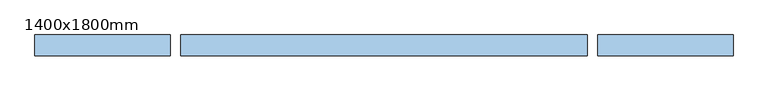
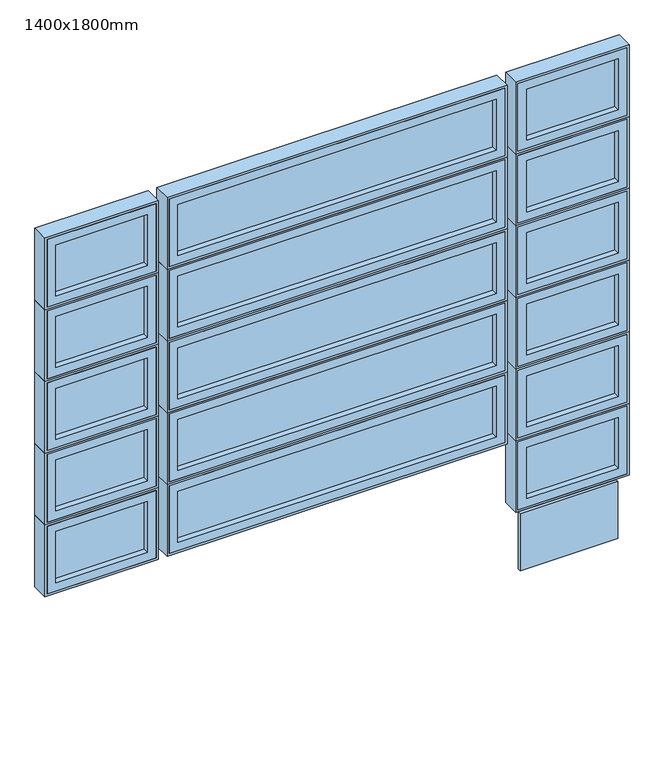
"""IFC4 building model written with IfcOpenShell, lengths in millimetres: window geometry, Janela Basculante 01 : 1400x1800mm."""

from ifc_helpers import new_model, si_unit, frame, origin, place, context, project, spatial, polyline, outline, extrude, faceted_brep, source, transform, mapped, element, save


def window_1400x1800mm_563ee437(model_context):
    return source(origin(), model_context, "Body", "SolidModel", [
        extrude(outline(polyline([(652.0, -29.6), (652.0, -36.6), (428.0, -36.6), (428.0, -29.6), (652.0, -29.6)])), frame((0.0, 0.0, 2164.0), z_axis=(0.0, 0.0, 1.0), x_axis=(1.0, 0.0, 0.0)), (0.0, 0.0, 1.0), 138.0),
        faceted_brep([(435.0, -50.6, 2295.0), (435.0, -50.6, 2171.0), (435.0, -36.6, 2171.0), (435.0, -36.6, 2295.0), (428.0, -36.6, 2302.0), (428.0, -36.6, 2164.0), (428.0, -29.6, 2164.0), (428.0, -29.6, 2302.0), (435.0, -29.6, 2295.0), (435.0, -29.6, 2171.0), (435.0, -15.6, 2171.0), (435.0, -15.6, 2295.0), (415.0, -15.6, 2315.0), (415.0, -15.6, 2151.0), (415.0, -50.6, 2151.0), (415.0, -50.6, 2315.0), (645.0, -50.6, 2171.0), (645.0, -36.6, 2171.0), (652.0, -36.6, 2164.0), (652.0, -29.6, 2164.0), (645.0, -29.6, 2171.0), (645.0, -15.6, 2171.0), (665.0, -15.6, 2151.0), (665.0, -50.6, 2151.0), (645.0, -50.6, 2295.0), (645.0, -36.6, 2295.0), (652.0, -36.6, 2302.0), (652.0, -29.6, 2302.0), (645.0, -29.6, 2295.0), (645.0, -15.6, 2295.0), (665.0, -15.6, 2315.0), (665.0, -50.6, 2315.0)], [[[0, 1, 2, 3]], [[4, 5, 6, 7]], [[8, 9, 10, 11]], [[12, 13, 14, 15]], [[1, 16, 17, 2]], [[5, 18, 19, 6]], [[9, 20, 21, 10]], [[13, 22, 23, 14]], [[16, 24, 25, 17]], [[18, 26, 27, 19]], [[20, 28, 29, 21]], [[22, 30, 31, 23]], [[15, 14, 23, 31], [1, 0, 24, 16]], [[24, 0, 3, 25]], [[5, 4, 26, 18], [3, 2, 17, 25]], [[26, 4, 7, 27]], [[7, 6, 19, 27], [9, 8, 28, 20]], [[28, 8, 11, 29]], [[13, 12, 30, 22], [11, 10, 21, 29]], [[30, 12, 15, 31]]]),
        faceted_brep([(415.0, -50.6, 2315.0), (415.0, -50.6, 2151.0), (415.0, -15.6, 2151.0), (415.0, -15.6, 2315.0), (420.0, -15.6, 2310.0), (420.0, -15.6, 2156.0), (420.0, -10.6, 2156.0), (420.0, -10.6, 2310.0), (410.0, -10.6, 2320.0), (410.0, -10.6, 2146.0), (410.0, -50.6, 2146.0), (410.0, -50.6, 2320.0), (665.0, -50.6, 2151.0), (665.0, -15.6, 2151.0), (660.0, -15.6, 2156.0), (660.0, -10.6, 2156.0), (670.0, -10.6, 2146.0), (670.0, -50.6, 2146.0), (665.0, -50.6, 2315.0), (665.0, -15.6, 2315.0), (660.0, -15.6, 2310.0), (660.0, -10.6, 2310.0), (670.0, -10.6, 2320.0), (670.0, -50.6, 2320.0)], [[[0, 1, 2, 3]], [[4, 5, 6, 7]], [[8, 9, 10, 11]], [[1, 12, 13, 2]], [[5, 14, 15, 6]], [[9, 16, 17, 10]], [[12, 18, 19, 13]], [[14, 20, 21, 15]], [[16, 22, 23, 17]], [[11, 10, 17, 23], [1, 0, 18, 12]], [[18, 0, 3, 19]], [[3, 2, 13, 19], [5, 4, 20, 14]], [[20, 4, 7, 21]], [[9, 8, 22, 16], [7, 6, 15, 21]], [[22, 8, 11, 23]]]),
        extrude(outline(polyline([(652.0, -29.6), (652.0, -36.6), (428.0, -36.6), (428.0, -29.6), (652.0, -29.6)])), frame((0.0, 0.0, 1990.0), z_axis=(0.0, 0.0, 1.0), x_axis=(1.0, 0.0, 0.0)), (0.0, 0.0, 1.0), 138.0),
        faceted_brep([(435.0, -50.6, 2121.0), (435.0, -50.6, 1997.0), (435.0, -36.6, 1997.0), (435.0, -36.6, 2121.0), (428.0, -36.6, 2128.0), (428.0, -36.6, 1990.0), (428.0, -29.6, 1990.0), (428.0, -29.6, 2128.0), (435.0, -29.6, 2121.0), (435.0, -29.6, 1997.0), (435.0, -15.6, 1997.0), (435.0, -15.6, 2121.0), (415.0, -15.6, 2141.0), (415.0, -15.6, 1977.0), (415.0, -50.6, 1977.0), (415.0, -50.6, 2141.0), (645.0, -50.6, 1997.0), (645.0, -36.6, 1997.0), (652.0, -36.6, 1990.0), (652.0, -29.6, 1990.0), (645.0, -29.6, 1997.0), (645.0, -15.6, 1997.0), (665.0, -15.6, 1977.0), (665.0, -50.6, 1977.0), (645.0, -50.6, 2121.0), (645.0, -36.6, 2121.0), (652.0, -36.6, 2128.0), (652.0, -29.6, 2128.0), (645.0, -29.6, 2121.0), (645.0, -15.6, 2121.0), (665.0, -15.6, 2141.0), (665.0, -50.6, 2141.0)], [[[0, 1, 2, 3]], [[4, 5, 6, 7]], [[8, 9, 10, 11]], [[12, 13, 14, 15]], [[1, 16, 17, 2]], [[5, 18, 19, 6]], [[9, 20, 21, 10]], [[13, 22, 23, 14]], [[16, 24, 25, 17]], [[18, 26, 27, 19]], [[20, 28, 29, 21]], [[22, 30, 31, 23]], [[15, 14, 23, 31], [1, 0, 24, 16]], [[24, 0, 3, 25]], [[5, 4, 26, 18], [3, 2, 17, 25]], [[26, 4, 7, 27]], [[7, 6, 19, 27], [9, 8, 28, 20]], [[28, 8, 11, 29]], [[13, 12, 30, 22], [11, 10, 21, 29]], [[30, 12, 15, 31]]]),
        faceted_brep([(415.0, -50.6, 2141.0), (415.0, -50.6, 1977.0), (415.0, -15.6, 1977.0), (415.0, -15.6, 2141.0), (420.0, -15.6, 2136.0), (420.0, -15.6, 1982.0), (420.0, -10.6, 1982.0), (420.0, -10.6, 2136.0), (410.0, -10.6, 2146.0), (410.0, -10.6, 1972.0), (410.0, -50.6, 1972.0), (410.0, -50.6, 2146.0), (665.0, -50.6, 1977.0), (665.0, -15.6, 1977.0), (660.0, -15.6, 1982.0), (660.0, -10.6, 1982.0), (670.0, -10.6, 1972.0), (670.0, -50.6, 1972.0), (665.0, -50.6, 2141.0), (665.0, -15.6, 2141.0), (660.0, -15.6, 2136.0), (660.0, -10.6, 2136.0), (670.0, -10.6, 2146.0), (670.0, -50.6, 2146.0)], [[[0, 1, 2, 3]], [[4, 5, 6, 7]], [[8, 9, 10, 11]], [[1, 12, 13, 2]], [[5, 14, 15, 6]], [[9, 16, 17, 10]], [[12, 18, 19, 13]], [[14, 20, 21, 15]], [[16, 22, 23, 17]], [[11, 10, 17, 23], [1, 0, 18, 12]], [[18, 0, 3, 19]], [[3, 2, 13, 19], [5, 4, 20, 14]], [[20, 4, 7, 21]], [[9, 8, 22, 16], [7, 6, 15, 21]], [[22, 8, 11, 23]]]),
        extrude(outline(polyline([(652.0, -29.6), (652.0, -36.6), (428.0, -36.6), (428.0, -29.6), (652.0, -29.6)])), frame((0.0, 0.0, 1816.0), z_axis=(0.0, 0.0, 1.0), x_axis=(1.0, 0.0, 0.0)), (0.0, 0.0, 1.0), 138.0),
        faceted_brep([(435.0, -50.6, 1947.0), (435.0, -50.6, 1823.0), (435.0, -36.6, 1823.0), (435.0, -36.6, 1947.0), (428.0, -36.6, 1954.0), (428.0, -36.6, 1816.0), (428.0, -29.6, 1816.0), (428.0, -29.6, 1954.0), (435.0, -29.6, 1947.0), (435.0, -29.6, 1823.0), (435.0, -15.6, 1823.0), (435.0, -15.6, 1947.0), (415.0, -15.6, 1967.0), (415.0, -15.6, 1803.0), (415.0, -50.6, 1803.0), (415.0, -50.6, 1967.0), (645.0, -50.6, 1823.0), (645.0, -36.6, 1823.0), (652.0, -36.6, 1816.0), (652.0, -29.6, 1816.0), (645.0, -29.6, 1823.0), (645.0, -15.6, 1823.0), (665.0, -15.6, 1803.0), (665.0, -50.6, 1803.0), (645.0, -50.6, 1947.0), (645.0, -36.6, 1947.0), (652.0, -36.6, 1954.0), (652.0, -29.6, 1954.0), (645.0, -29.6, 1947.0), (645.0, -15.6, 1947.0), (665.0, -15.6, 1967.0), (665.0, -50.6, 1967.0)], [[[0, 1, 2, 3]], [[4, 5, 6, 7]], [[8, 9, 10, 11]], [[12, 13, 14, 15]], [[1, 16, 17, 2]], [[5, 18, 19, 6]], [[9, 20, 21, 10]], [[13, 22, 23, 14]], [[16, 24, 25, 17]], [[18, 26, 27, 19]], [[20, 28, 29, 21]], [[22, 30, 31, 23]], [[15, 14, 23, 31], [1, 0, 24, 16]], [[24, 0, 3, 25]], [[5, 4, 26, 18], [3, 2, 17, 25]], [[26, 4, 7, 27]], [[7, 6, 19, 27], [9, 8, 28, 20]], [[28, 8, 11, 29]], [[13, 12, 30, 22], [11, 10, 21, 29]], [[30, 12, 15, 31]]]),
        faceted_brep([(415.0, -50.6, 1967.0), (415.0, -50.6, 1803.0), (415.0, -15.6, 1803.0), (415.0, -15.6, 1967.0), (420.0, -15.6, 1962.0), (420.0, -15.6, 1808.0), (420.0, -10.6, 1808.0), (420.0, -10.6, 1962.0), (410.0, -10.6, 1972.0), (410.0, -10.6, 1798.0), (410.0, -50.6, 1798.0), (410.0, -50.6, 1972.0), (665.0, -50.6, 1803.0), (665.0, -15.6, 1803.0), (660.0, -15.6, 1808.0), (660.0, -10.6, 1808.0), (670.0, -10.6, 1798.0), (670.0, -50.6, 1798.0), (665.0, -50.6, 1967.0), (665.0, -15.6, 1967.0), (660.0, -15.6, 1962.0), (660.0, -10.6, 1962.0), (670.0, -10.6, 1972.0), (670.0, -50.6, 1972.0)], [[[0, 1, 2, 3]], [[4, 5, 6, 7]], [[8, 9, 10, 11]], [[1, 12, 13, 2]], [[5, 14, 15, 6]], [[9, 16, 17, 10]], [[12, 18, 19, 13]], [[14, 20, 21, 15]], [[16, 22, 23, 17]], [[11, 10, 17, 23], [1, 0, 18, 12]], [[18, 0, 3, 19]], [[3, 2, 13, 19], [5, 4, 20, 14]], [[20, 4, 7, 21]], [[9, 8, 22, 16], [7, 6, 15, 21]], [[22, 8, 11, 23]]]),
        extrude(outline(polyline([(-372.0, -29.6), (372.0, -29.6), (372.0, -36.6), (-372.0, -36.6), (-372.0, -29.6)])), frame((0.0, 0.0, 2164.0), z_axis=(0.0, 0.0, 1.0), x_axis=(1.0, 0.0, 0.0)), (0.0, 0.0, 1.0), 138.0),
        faceted_brep([(365.0, -50.6, 2295.0), (365.0, -36.6, 2295.0), (365.0, -36.6, 2171.0), (365.0, -50.6, 2171.0), (372.0, -36.6, 2302.0), (372.0, -29.6, 2302.0), (372.0, -29.6, 2164.0), (372.0, -36.6, 2164.0), (365.0, -29.6, 2295.0), (365.0, -15.6, 2295.0), (365.0, -15.6, 2171.0), (365.0, -29.6, 2171.0), (385.0, -15.6, 2315.0), (385.0, -50.6, 2315.0), (385.0, -50.6, 2151.0), (385.0, -15.6, 2151.0), (-365.0, -36.6, 2171.0), (-365.0, -50.6, 2171.0), (-372.0, -29.6, 2164.0), (-372.0, -36.6, 2164.0), (-365.0, -15.6, 2171.0), (-365.0, -29.6, 2171.0), (-385.0, -50.6, 2151.0), (-385.0, -15.6, 2151.0), (-365.0, -36.6, 2295.0), (-365.0, -50.6, 2295.0), (-372.0, -29.6, 2302.0), (-372.0, -36.6, 2302.0), (-365.0, -15.6, 2295.0), (-365.0, -29.6, 2295.0), (-385.0, -50.6, 2315.0), (-385.0, -15.6, 2315.0)], [[[0, 1, 2, 3]], [[4, 5, 6, 7]], [[8, 9, 10, 11]], [[12, 13, 14, 15]], [[3, 2, 16, 17]], [[7, 6, 18, 19]], [[11, 10, 20, 21]], [[15, 14, 22, 23]], [[17, 16, 24, 25]], [[19, 18, 26, 27]], [[21, 20, 28, 29]], [[23, 22, 30, 31]], [[13, 30, 22, 14], [3, 17, 25, 0]], [[25, 24, 1, 0]], [[7, 19, 27, 4], [1, 24, 16, 2]], [[27, 26, 5, 4]], [[5, 26, 18, 6], [11, 21, 29, 8]], [[29, 28, 9, 8]], [[15, 23, 31, 12], [9, 28, 20, 10]], [[31, 30, 13, 12]]]),
        faceted_brep([(385.0, -50.6, 2315.0), (385.0, -15.6, 2315.0), (385.0, -15.6, 2151.0), (385.0, -50.6, 2151.0), (380.0, -15.6, 2310.0), (380.0, -10.6, 2310.0), (380.0, -10.6, 2156.0), (380.0, -15.6, 2156.0), (390.0, -10.6, 2320.0), (390.0, -50.6, 2320.0), (390.0, -50.6, 2146.0), (390.0, -10.6, 2146.0), (-385.0, -15.6, 2151.0), (-385.0, -50.6, 2151.0), (-380.0, -10.6, 2156.0), (-380.0, -15.6, 2156.0), (-390.0, -50.6, 2146.0), (-390.0, -10.6, 2146.0), (-385.0, -15.6, 2315.0), (-385.0, -50.6, 2315.0), (-380.0, -10.6, 2310.0), (-380.0, -15.6, 2310.0), (-390.0, -50.6, 2320.0), (-390.0, -10.6, 2320.0)], [[[0, 1, 2, 3]], [[4, 5, 6, 7]], [[8, 9, 10, 11]], [[3, 2, 12, 13]], [[7, 6, 14, 15]], [[11, 10, 16, 17]], [[13, 12, 18, 19]], [[15, 14, 20, 21]], [[17, 16, 22, 23]], [[9, 22, 16, 10], [3, 13, 19, 0]], [[19, 18, 1, 0]], [[1, 18, 12, 2], [7, 15, 21, 4]], [[21, 20, 5, 4]], [[11, 17, 23, 8], [5, 20, 14, 6]], [[23, 22, 9, 8]]]),
        extrude(outline(polyline([(-372.0, -29.6), (372.0, -29.6), (372.0, -36.6), (-372.0, -36.6), (-372.0, -29.6)])), frame((0.0, 0.0, 1990.0), z_axis=(0.0, 0.0, 1.0), x_axis=(1.0, 0.0, 0.0)), (0.0, 0.0, 1.0), 138.0),
        faceted_brep([(365.0, -50.6, 2121.0), (365.0, -36.6, 2121.0), (365.0, -36.6, 1997.0), (365.0, -50.6, 1997.0), (372.0, -36.6, 2128.0), (372.0, -29.6, 2128.0), (372.0, -29.6, 1990.0), (372.0, -36.6, 1990.0), (365.0, -29.6, 2121.0), (365.0, -15.6, 2121.0), (365.0, -15.6, 1997.0), (365.0, -29.6, 1997.0), (385.0, -15.6, 2141.0), (385.0, -50.6, 2141.0), (385.0, -50.6, 1977.0), (385.0, -15.6, 1977.0), (-365.0, -36.6, 1997.0), (-365.0, -50.6, 1997.0), (-372.0, -29.6, 1990.0), (-372.0, -36.6, 1990.0), (-365.0, -15.6, 1997.0), (-365.0, -29.6, 1997.0), (-385.0, -50.6, 1977.0), (-385.0, -15.6, 1977.0), (-365.0, -36.6, 2121.0), (-365.0, -50.6, 2121.0), (-372.0, -29.6, 2128.0), (-372.0, -36.6, 2128.0), (-365.0, -15.6, 2121.0), (-365.0, -29.6, 2121.0), (-385.0, -50.6, 2141.0), (-385.0, -15.6, 2141.0)], [[[0, 1, 2, 3]], [[4, 5, 6, 7]], [[8, 9, 10, 11]], [[12, 13, 14, 15]], [[3, 2, 16, 17]], [[7, 6, 18, 19]], [[11, 10, 20, 21]], [[15, 14, 22, 23]], [[17, 16, 24, 25]], [[19, 18, 26, 27]], [[21, 20, 28, 29]], [[23, 22, 30, 31]], [[13, 30, 22, 14], [3, 17, 25, 0]], [[25, 24, 1, 0]], [[7, 19, 27, 4], [1, 24, 16, 2]], [[27, 26, 5, 4]], [[5, 26, 18, 6], [11, 21, 29, 8]], [[29, 28, 9, 8]], [[15, 23, 31, 12], [9, 28, 20, 10]], [[31, 30, 13, 12]]]),
        faceted_brep([(385.0, -50.6, 2141.0), (385.0, -15.6, 2141.0), (385.0, -15.6, 1977.0), (385.0, -50.6, 1977.0), (380.0, -15.6, 2136.0), (380.0, -10.6, 2136.0), (380.0, -10.6, 1982.0), (380.0, -15.6, 1982.0), (390.0, -10.6, 2146.0), (390.0, -50.6, 2146.0), (390.0, -50.6, 1972.0), (390.0, -10.6, 1972.0), (-385.0, -15.6, 1977.0), (-385.0, -50.6, 1977.0), (-380.0, -10.6, 1982.0), (-380.0, -15.6, 1982.0), (-390.0, -50.6, 1972.0), (-390.0, -10.6, 1972.0), (-385.0, -15.6, 2141.0), (-385.0, -50.6, 2141.0), (-380.0, -10.6, 2136.0), (-380.0, -15.6, 2136.0), (-390.0, -50.6, 2146.0), (-390.0, -10.6, 2146.0)], [[[0, 1, 2, 3]], [[4, 5, 6, 7]], [[8, 9, 10, 11]], [[3, 2, 12, 13]], [[7, 6, 14, 15]], [[11, 10, 16, 17]], [[13, 12, 18, 19]], [[15, 14, 20, 21]], [[17, 16, 22, 23]], [[9, 22, 16, 10], [3, 13, 19, 0]], [[19, 18, 1, 0]], [[1, 18, 12, 2], [7, 15, 21, 4]], [[21, 20, 5, 4]], [[11, 17, 23, 8], [5, 20, 14, 6]], [[23, 22, 9, 8]]]),
        extrude(outline(polyline([(-372.0, -29.6), (372.0, -29.6), (372.0, -36.6), (-372.0, -36.6), (-372.0, -29.6)])), frame((0.0, 0.0, 1816.0), z_axis=(0.0, 0.0, 1.0), x_axis=(1.0, 0.0, 0.0)), (0.0, 0.0, 1.0), 138.0),
        faceted_brep([(365.0, -50.6, 1947.0), (365.0, -36.6, 1947.0), (365.0, -36.6, 1823.0), (365.0, -50.6, 1823.0), (372.0, -36.6, 1954.0), (372.0, -29.6, 1954.0), (372.0, -29.6, 1816.0), (372.0, -36.6, 1816.0), (365.0, -29.6, 1947.0), (365.0, -15.6, 1947.0), (365.0, -15.6, 1823.0), (365.0, -29.6, 1823.0), (385.0, -15.6, 1967.0), (385.0, -50.6, 1967.0), (385.0, -50.6, 1803.0), (385.0, -15.6, 1803.0), (-365.0, -36.6, 1823.0), (-365.0, -50.6, 1823.0), (-372.0, -29.6, 1816.0), (-372.0, -36.6, 1816.0), (-365.0, -15.6, 1823.0), (-365.0, -29.6, 1823.0), (-385.0, -50.6, 1803.0), (-385.0, -15.6, 1803.0), (-365.0, -36.6, 1947.0), (-365.0, -50.6, 1947.0), (-372.0, -29.6, 1954.0), (-372.0, -36.6, 1954.0), (-365.0, -15.6, 1947.0), (-365.0, -29.6, 1947.0), (-385.0, -50.6, 1967.0), (-385.0, -15.6, 1967.0)], [[[0, 1, 2, 3]], [[4, 5, 6, 7]], [[8, 9, 10, 11]], [[12, 13, 14, 15]], [[3, 2, 16, 17]], [[7, 6, 18, 19]], [[11, 10, 20, 21]], [[15, 14, 22, 23]], [[17, 16, 24, 25]], [[19, 18, 26, 27]], [[21, 20, 28, 29]], [[23, 22, 30, 31]], [[13, 30, 22, 14], [3, 17, 25, 0]], [[25, 24, 1, 0]], [[7, 19, 27, 4], [1, 24, 16, 2]], [[27, 26, 5, 4]], [[5, 26, 18, 6], [11, 21, 29, 8]], [[29, 28, 9, 8]], [[15, 23, 31, 12], [9, 28, 20, 10]], [[31, 30, 13, 12]]]),
        faceted_brep([(385.0, -50.6, 1967.0), (385.0, -15.6, 1967.0), (385.0, -15.6, 1803.0), (385.0, -50.6, 1803.0), (380.0, -15.6, 1962.0), (380.0, -10.6, 1962.0), (380.0, -10.6, 1808.0), (380.0, -15.6, 1808.0), (390.0, -10.6, 1972.0), (390.0, -50.6, 1972.0), (390.0, -50.6, 1798.0), (390.0, -10.6, 1798.0), (-385.0, -15.6, 1803.0), (-385.0, -50.6, 1803.0), (-380.0, -10.6, 1808.0), (-380.0, -15.6, 1808.0), (-390.0, -50.6, 1798.0), (-390.0, -10.6, 1798.0), (-385.0, -15.6, 1967.0), (-385.0, -50.6, 1967.0), (-380.0, -10.6, 1962.0), (-380.0, -15.6, 1962.0), (-390.0, -50.6, 1972.0), (-390.0, -10.6, 1972.0)], [[[0, 1, 2, 3]], [[4, 5, 6, 7]], [[8, 9, 10, 11]], [[3, 2, 12, 13]], [[7, 6, 14, 15]], [[11, 10, 16, 17]], [[13, 12, 18, 19]], [[15, 14, 20, 21]], [[17, 16, 22, 23]], [[9, 22, 16, 10], [3, 13, 19, 0]], [[19, 18, 1, 0]], [[1, 18, 12, 2], [7, 15, 21, 4]], [[21, 20, 5, 4]], [[11, 17, 23, 8], [5, 20, 14, 6]], [[23, 22, 9, 8]]]),
        extrude(outline(polyline([(-428.0, -29.6), (-428.0, -36.6), (-652.0, -36.6), (-652.0, -29.6), (-428.0, -29.6)])), frame((0.0, 0.0, 2164.0), z_axis=(0.0, 0.0, 1.0), x_axis=(1.0, 0.0, 0.0)), (0.0, 0.0, 1.0), 138.0),
        faceted_brep([(-645.0, -50.6, 2295.0), (-645.0, -50.6, 2171.0), (-645.0, -36.6, 2171.0), (-645.0, -36.6, 2295.0), (-652.0, -36.6, 2302.0), (-652.0, -36.6, 2164.0), (-652.0, -29.6, 2164.0), (-652.0, -29.6, 2302.0), (-645.0, -29.6, 2295.0), (-645.0, -29.6, 2171.0), (-645.0, -15.6, 2171.0), (-645.0, -15.6, 2295.0), (-665.0, -15.6, 2315.0), (-665.0, -15.6, 2151.0), (-665.0, -50.6, 2151.0), (-665.0, -50.6, 2315.0), (-435.0, -50.6, 2171.0), (-435.0, -36.6, 2171.0), (-428.0, -36.6, 2164.0), (-428.0, -29.6, 2164.0), (-435.0, -29.6, 2171.0), (-435.0, -15.6, 2171.0), (-415.0, -15.6, 2151.0), (-415.0, -50.6, 2151.0), (-435.0, -50.6, 2295.0), (-435.0, -36.6, 2295.0), (-428.0, -36.6, 2302.0), (-428.0, -29.6, 2302.0), (-435.0, -29.6, 2295.0), (-435.0, -15.6, 2295.0), (-415.0, -15.6, 2315.0), (-415.0, -50.6, 2315.0)], [[[0, 1, 2, 3]], [[4, 5, 6, 7]], [[8, 9, 10, 11]], [[12, 13, 14, 15]], [[1, 16, 17, 2]], [[5, 18, 19, 6]], [[9, 20, 21, 10]], [[13, 22, 23, 14]], [[16, 24, 25, 17]], [[18, 26, 27, 19]], [[20, 28, 29, 21]], [[22, 30, 31, 23]], [[15, 14, 23, 31], [1, 0, 24, 16]], [[24, 0, 3, 25]], [[5, 4, 26, 18], [3, 2, 17, 25]], [[26, 4, 7, 27]], [[7, 6, 19, 27], [9, 8, 28, 20]], [[28, 8, 11, 29]], [[13, 12, 30, 22], [11, 10, 21, 29]], [[30, 12, 15, 31]]]),
        faceted_brep([(-665.0, -50.6, 2315.0), (-665.0, -50.6, 2151.0), (-665.0, -15.6, 2151.0), (-665.0, -15.6, 2315.0), (-660.0, -15.6, 2310.0), (-660.0, -15.6, 2156.0), (-660.0, -10.6, 2156.0), (-660.0, -10.6, 2310.0), (-670.0, -10.6, 2320.0), (-670.0, -10.6, 2146.0), (-670.0, -50.6, 2146.0), (-670.0, -50.6, 2320.0), (-415.0, -50.6, 2151.0), (-415.0, -15.6, 2151.0), (-420.0, -15.6, 2156.0), (-420.0, -10.6, 2156.0), (-410.0, -10.6, 2146.0), (-410.0, -50.6, 2146.0), (-415.0, -50.6, 2315.0), (-415.0, -15.6, 2315.0), (-420.0, -15.6, 2310.0), (-420.0, -10.6, 2310.0), (-410.0, -10.6, 2320.0), (-410.0, -50.6, 2320.0)], [[[0, 1, 2, 3]], [[4, 5, 6, 7]], [[8, 9, 10, 11]], [[1, 12, 13, 2]], [[5, 14, 15, 6]], [[9, 16, 17, 10]], [[12, 18, 19, 13]], [[14, 20, 21, 15]], [[16, 22, 23, 17]], [[11, 10, 17, 23], [1, 0, 18, 12]], [[18, 0, 3, 19]], [[3, 2, 13, 19], [5, 4, 20, 14]], [[20, 4, 7, 21]], [[9, 8, 22, 16], [7, 6, 15, 21]], [[22, 8, 11, 23]]]),
        extrude(outline(polyline([(-428.0, -29.6), (-428.0, -36.6), (-652.0, -36.6), (-652.0, -29.6), (-428.0, -29.6)])), frame((0.0, 0.0, 1990.0), z_axis=(0.0, 0.0, 1.0), x_axis=(1.0, 0.0, 0.0)), (0.0, 0.0, 1.0), 138.0),
        faceted_brep([(-645.0, -50.6, 2121.0), (-645.0, -50.6, 1997.0), (-645.0, -36.6, 1997.0), (-645.0, -36.6, 2121.0), (-652.0, -36.6, 2128.0), (-652.0, -36.6, 1990.0), (-652.0, -29.6, 1990.0), (-652.0, -29.6, 2128.0), (-645.0, -29.6, 2121.0), (-645.0, -29.6, 1997.0), (-645.0, -15.6, 1997.0), (-645.0, -15.6, 2121.0), (-665.0, -15.6, 2141.0), (-665.0, -15.6, 1977.0), (-665.0, -50.6, 1977.0), (-665.0, -50.6, 2141.0), (-435.0, -50.6, 1997.0), (-435.0, -36.6, 1997.0), (-428.0, -36.6, 1990.0), (-428.0, -29.6, 1990.0), (-435.0, -29.6, 1997.0), (-435.0, -15.6, 1997.0), (-415.0, -15.6, 1977.0), (-415.0, -50.6, 1977.0), (-435.0, -50.6, 2121.0), (-435.0, -36.6, 2121.0), (-428.0, -36.6, 2128.0), (-428.0, -29.6, 2128.0), (-435.0, -29.6, 2121.0), (-435.0, -15.6, 2121.0), (-415.0, -15.6, 2141.0), (-415.0, -50.6, 2141.0)], [[[0, 1, 2, 3]], [[4, 5, 6, 7]], [[8, 9, 10, 11]], [[12, 13, 14, 15]], [[1, 16, 17, 2]], [[5, 18, 19, 6]], [[9, 20, 21, 10]], [[13, 22, 23, 14]], [[16, 24, 25, 17]], [[18, 26, 27, 19]], [[20, 28, 29, 21]], [[22, 30, 31, 23]], [[15, 14, 23, 31], [1, 0, 24, 16]], [[24, 0, 3, 25]], [[5, 4, 26, 18], [3, 2, 17, 25]], [[26, 4, 7, 27]], [[7, 6, 19, 27], [9, 8, 28, 20]], [[28, 8, 11, 29]], [[13, 12, 30, 22], [11, 10, 21, 29]], [[30, 12, 15, 31]]]),
        faceted_brep([(-665.0, -50.6, 2141.0), (-665.0, -50.6, 1977.0), (-665.0, -15.6, 1977.0), (-665.0, -15.6, 2141.0), (-660.0, -15.6, 2136.0), (-660.0, -15.6, 1982.0), (-660.0, -10.6, 1982.0), (-660.0, -10.6, 2136.0), (-670.0, -10.6, 2146.0), (-670.0, -10.6, 1972.0), (-670.0, -50.6, 1972.0), (-670.0, -50.6, 2146.0), (-415.0, -50.6, 1977.0), (-415.0, -15.6, 1977.0), (-420.0, -15.6, 1982.0), (-420.0, -10.6, 1982.0), (-410.0, -10.6, 1972.0), (-410.0, -50.6, 1972.0), (-415.0, -50.6, 2141.0), (-415.0, -15.6, 2141.0), (-420.0, -15.6, 2136.0), (-420.0, -10.6, 2136.0), (-410.0, -10.6, 2146.0), (-410.0, -50.6, 2146.0)], [[[0, 1, 2, 3]], [[4, 5, 6, 7]], [[8, 9, 10, 11]], [[1, 12, 13, 2]], [[5, 14, 15, 6]], [[9, 16, 17, 10]], [[12, 18, 19, 13]], [[14, 20, 21, 15]], [[16, 22, 23, 17]], [[11, 10, 17, 23], [1, 0, 18, 12]], [[18, 0, 3, 19]], [[3, 2, 13, 19], [5, 4, 20, 14]], [[20, 4, 7, 21]], [[9, 8, 22, 16], [7, 6, 15, 21]], [[22, 8, 11, 23]]]),
        extrude(outline(polyline([(-428.0, -29.6), (-428.0, -36.6), (-652.0, -36.6), (-652.0, -29.6), (-428.0, -29.6)])), frame((0.0, 0.0, 1816.0), z_axis=(0.0, 0.0, 1.0), x_axis=(1.0, 0.0, 0.0)), (0.0, 0.0, 1.0), 138.0),
        faceted_brep([(-645.0, -50.6, 1947.0), (-645.0, -50.6, 1823.0), (-645.0, -36.6, 1823.0), (-645.0, -36.6, 1947.0), (-652.0, -36.6, 1954.0), (-652.0, -36.6, 1816.0), (-652.0, -29.6, 1816.0), (-652.0, -29.6, 1954.0), (-645.0, -29.6, 1947.0), (-645.0, -29.6, 1823.0), (-645.0, -15.6, 1823.0), (-645.0, -15.6, 1947.0), (-665.0, -15.6, 1967.0), (-665.0, -15.6, 1803.0), (-665.0, -50.6, 1803.0), (-665.0, -50.6, 1967.0), (-435.0, -50.6, 1823.0), (-435.0, -36.6, 1823.0), (-428.0, -36.6, 1816.0), (-428.0, -29.6, 1816.0), (-435.0, -29.6, 1823.0), (-435.0, -15.6, 1823.0), (-415.0, -15.6, 1803.0), (-415.0, -50.6, 1803.0), (-435.0, -50.6, 1947.0), (-435.0, -36.6, 1947.0), (-428.0, -36.6, 1954.0), (-428.0, -29.6, 1954.0), (-435.0, -29.6, 1947.0), (-435.0, -15.6, 1947.0), (-415.0, -15.6, 1967.0), (-415.0, -50.6, 1967.0)], [[[0, 1, 2, 3]], [[4, 5, 6, 7]], [[8, 9, 10, 11]], [[12, 13, 14, 15]], [[1, 16, 17, 2]], [[5, 18, 19, 6]], [[9, 20, 21, 10]], [[13, 22, 23, 14]], [[16, 24, 25, 17]], [[18, 26, 27, 19]], [[20, 28, 29, 21]], [[22, 30, 31, 23]], [[15, 14, 23, 31], [1, 0, 24, 16]], [[24, 0, 3, 25]], [[5, 4, 26, 18], [3, 2, 17, 25]], [[26, 4, 7, 27]], [[7, 6, 19, 27], [9, 8, 28, 20]], [[28, 8, 11, 29]], [[13, 12, 30, 22], [11, 10, 21, 29]], [[30, 12, 15, 31]]]),
        faceted_brep([(-665.0, -50.6, 1967.0), (-665.0, -50.6, 1803.0), (-665.0, -15.6, 1803.0), (-665.0, -15.6, 1967.0), (-660.0, -15.6, 1962.0), (-660.0, -15.6, 1808.0), (-660.0, -10.6, 1808.0), (-660.0, -10.6, 1962.0), (-670.0, -10.6, 1972.0), (-670.0, -10.6, 1798.0), (-670.0, -50.6, 1798.0), (-670.0, -50.6, 1972.0), (-415.0, -50.6, 1803.0), (-415.0, -15.6, 1803.0), (-420.0, -15.6, 1808.0), (-420.0, -10.6, 1808.0), (-410.0, -10.6, 1798.0), (-410.0, -50.6, 1798.0), (-415.0, -50.6, 1967.0), (-415.0, -15.6, 1967.0), (-420.0, -15.6, 1962.0), (-420.0, -10.6, 1962.0), (-410.0, -10.6, 1972.0), (-410.0, -50.6, 1972.0)], [[[0, 1, 2, 3]], [[4, 5, 6, 7]], [[8, 9, 10, 11]], [[1, 12, 13, 2]], [[5, 14, 15, 6]], [[9, 16, 17, 10]], [[12, 18, 19, 13]], [[14, 20, 21, 15]], [[16, 22, 23, 17]], [[11, 10, 17, 23], [1, 0, 18, 12]], [[18, 0, 3, 19]], [[3, 2, 13, 19], [5, 4, 20, 14]], [[20, 4, 7, 21]], [[9, 8, 22, 16], [7, 6, 15, 21]], [[22, 8, 11, 23]]]),
        extrude(outline(polyline([(652.0, -29.6), (652.0, -36.6), (428.0, -36.6), (428.0, -29.6), (652.0, -29.6)])), frame((0.0, 0.0, 1642.0), z_axis=(0.0, 0.0, 1.0), x_axis=(1.0, 0.0, 0.0)), (0.0, 0.0, 1.0), 138.0),
        faceted_brep([(435.0, -50.6, 1773.0), (435.0, -50.6, 1649.0), (435.0, -36.6, 1649.0), (435.0, -36.6, 1773.0), (428.0, -36.6, 1780.0), (428.0, -36.6, 1642.0), (428.0, -29.6, 1642.0), (428.0, -29.6, 1780.0), (435.0, -29.6, 1773.0), (435.0, -29.6, 1649.0), (435.0, -15.6, 1649.0), (435.0, -15.6, 1773.0), (415.0, -15.6, 1793.0), (415.0, -15.6, 1629.0), (415.0, -50.6, 1629.0), (415.0, -50.6, 1793.0), (645.0, -50.6, 1649.0), (645.0, -36.6, 1649.0), (652.0, -36.6, 1642.0), (652.0, -29.6, 1642.0), (645.0, -29.6, 1649.0), (645.0, -15.6, 1649.0), (665.0, -15.6, 1629.0), (665.0, -50.6, 1629.0), (645.0, -50.6, 1773.0), (645.0, -36.6, 1773.0), (652.0, -36.6, 1780.0), (652.0, -29.6, 1780.0), (645.0, -29.6, 1773.0), (645.0, -15.6, 1773.0), (665.0, -15.6, 1793.0), (665.0, -50.6, 1793.0)], [[[0, 1, 2, 3]], [[4, 5, 6, 7]], [[8, 9, 10, 11]], [[12, 13, 14, 15]], [[1, 16, 17, 2]], [[5, 18, 19, 6]], [[9, 20, 21, 10]], [[13, 22, 23, 14]], [[16, 24, 25, 17]], [[18, 26, 27, 19]], [[20, 28, 29, 21]], [[22, 30, 31, 23]], [[15, 14, 23, 31], [1, 0, 24, 16]], [[24, 0, 3, 25]], [[5, 4, 26, 18], [3, 2, 17, 25]], [[26, 4, 7, 27]], [[7, 6, 19, 27], [9, 8, 28, 20]], [[28, 8, 11, 29]], [[13, 12, 30, 22], [11, 10, 21, 29]], [[30, 12, 15, 31]]]),
        faceted_brep([(415.0, -50.6, 1793.0), (415.0, -50.6, 1629.0), (415.0, -15.6, 1629.0), (415.0, -15.6, 1793.0), (420.0, -15.6, 1788.0), (420.0, -15.6, 1634.0), (420.0, -10.6, 1634.0), (420.0, -10.6, 1788.0), (410.0, -10.6, 1798.0), (410.0, -10.6, 1624.0), (410.0, -50.6, 1624.0), (410.0, -50.6, 1798.0), (665.0, -50.6, 1629.0), (665.0, -15.6, 1629.0), (660.0, -15.6, 1634.0), (660.0, -10.6, 1634.0), (670.0, -10.6, 1624.0), (670.0, -50.6, 1624.0), (665.0, -50.6, 1793.0), (665.0, -15.6, 1793.0), (660.0, -15.6, 1788.0), (660.0, -10.6, 1788.0), (670.0, -10.6, 1798.0), (670.0, -50.6, 1798.0)], [[[0, 1, 2, 3]], [[4, 5, 6, 7]], [[8, 9, 10, 11]], [[1, 12, 13, 2]], [[5, 14, 15, 6]], [[9, 16, 17, 10]], [[12, 18, 19, 13]], [[14, 20, 21, 15]], [[16, 22, 23, 17]], [[11, 10, 17, 23], [1, 0, 18, 12]], [[18, 0, 3, 19]], [[3, 2, 13, 19], [5, 4, 20, 14]], [[20, 4, 7, 21]], [[9, 8, 22, 16], [7, 6, 15, 21]], [[22, 8, 11, 23]]]),
        extrude(outline(polyline([(652.0, -29.6), (652.0, -36.6), (428.0, -36.6), (428.0, -29.6), (652.0, -29.6)])), frame((0.0, 0.0, 1468.0), z_axis=(0.0, 0.0, 1.0), x_axis=(1.0, 0.0, 0.0)), (0.0, 0.0, 1.0), 138.0),
        faceted_brep([(435.0, -50.6, 1599.0), (435.0, -50.6, 1475.0), (435.0, -36.6, 1475.0), (435.0, -36.6, 1599.0), (428.0, -36.6, 1606.0), (428.0, -36.6, 1468.0), (428.0, -29.6, 1468.0), (428.0, -29.6, 1606.0), (435.0, -29.6, 1599.0), (435.0, -29.6, 1475.0), (435.0, -15.6, 1475.0), (435.0, -15.6, 1599.0), (415.0, -15.6, 1619.0), (415.0, -15.6, 1455.0), (415.0, -50.6, 1455.0), (415.0, -50.6, 1619.0), (645.0, -50.6, 1475.0), (645.0, -36.6, 1475.0), (652.0, -36.6, 1468.0), (652.0, -29.6, 1468.0), (645.0, -29.6, 1475.0), (645.0, -15.6, 1475.0), (665.0, -15.6, 1455.0), (665.0, -50.6, 1455.0), (645.0, -50.6, 1599.0), (645.0, -36.6, 1599.0), (652.0, -36.6, 1606.0), (652.0, -29.6, 1606.0), (645.0, -29.6, 1599.0), (645.0, -15.6, 1599.0), (665.0, -15.6, 1619.0), (665.0, -50.6, 1619.0)], [[[0, 1, 2, 3]], [[4, 5, 6, 7]], [[8, 9, 10, 11]], [[12, 13, 14, 15]], [[1, 16, 17, 2]], [[5, 18, 19, 6]], [[9, 20, 21, 10]], [[13, 22, 23, 14]], [[16, 24, 25, 17]], [[18, 26, 27, 19]], [[20, 28, 29, 21]], [[22, 30, 31, 23]], [[15, 14, 23, 31], [1, 0, 24, 16]], [[24, 0, 3, 25]], [[5, 4, 26, 18], [3, 2, 17, 25]], [[26, 4, 7, 27]], [[7, 6, 19, 27], [9, 8, 28, 20]], [[28, 8, 11, 29]], [[13, 12, 30, 22], [11, 10, 21, 29]], [[30, 12, 15, 31]]]),
        faceted_brep([(415.0, -50.6, 1619.0), (415.0, -50.6, 1455.0), (415.0, -15.6, 1455.0), (415.0, -15.6, 1619.0), (420.0, -15.6, 1614.0), (420.0, -15.6, 1460.0), (420.0, -10.6, 1460.0), (420.0, -10.6, 1614.0), (410.0, -10.6, 1624.0), (410.0, -10.6, 1450.0), (410.0, -50.6, 1450.0), (410.0, -50.6, 1624.0), (665.0, -50.6, 1455.0), (665.0, -15.6, 1455.0), (660.0, -15.6, 1460.0), (660.0, -10.6, 1460.0), (670.0, -10.6, 1450.0), (670.0, -50.6, 1450.0), (665.0, -50.6, 1619.0), (665.0, -15.6, 1619.0), (660.0, -15.6, 1614.0), (660.0, -10.6, 1614.0), (670.0, -10.6, 1624.0), (670.0, -50.6, 1624.0)], [[[0, 1, 2, 3]], [[4, 5, 6, 7]], [[8, 9, 10, 11]], [[1, 12, 13, 2]], [[5, 14, 15, 6]], [[9, 16, 17, 10]], [[12, 18, 19, 13]], [[14, 20, 21, 15]], [[16, 22, 23, 17]], [[11, 10, 17, 23], [1, 0, 18, 12]], [[18, 0, 3, 19]], [[3, 2, 13, 19], [5, 4, 20, 14]], [[20, 4, 7, 21]], [[9, 8, 22, 16], [7, 6, 15, 21]], [[22, 8, 11, 23]]]),
        extrude(outline(polyline([(-372.0, -29.6), (372.0, -29.6), (372.0, -36.6), (-372.0, -36.6), (-372.0, -29.6)])), frame((0.0, 0.0, 1642.0), z_axis=(0.0, 0.0, 1.0), x_axis=(1.0, 0.0, 0.0)), (0.0, 0.0, 1.0), 138.0),
        faceted_brep([(365.0, -50.6, 1773.0), (365.0, -36.6, 1773.0), (365.0, -36.6, 1649.0), (365.0, -50.6, 1649.0), (372.0, -36.6, 1780.0), (372.0, -29.6, 1780.0), (372.0, -29.6, 1642.0), (372.0, -36.6, 1642.0), (365.0, -29.6, 1773.0), (365.0, -15.6, 1773.0), (365.0, -15.6, 1649.0), (365.0, -29.6, 1649.0), (385.0, -15.6, 1793.0), (385.0, -50.6, 1793.0), (385.0, -50.6, 1629.0), (385.0, -15.6, 1629.0), (-365.0, -36.6, 1649.0), (-365.0, -50.6, 1649.0), (-372.0, -29.6, 1642.0), (-372.0, -36.6, 1642.0), (-365.0, -15.6, 1649.0), (-365.0, -29.6, 1649.0), (-385.0, -50.6, 1629.0), (-385.0, -15.6, 1629.0), (-365.0, -36.6, 1773.0), (-365.0, -50.6, 1773.0), (-372.0, -29.6, 1780.0), (-372.0, -36.6, 1780.0), (-365.0, -15.6, 1773.0), (-365.0, -29.6, 1773.0), (-385.0, -50.6, 1793.0), (-385.0, -15.6, 1793.0)], [[[0, 1, 2, 3]], [[4, 5, 6, 7]], [[8, 9, 10, 11]], [[12, 13, 14, 15]], [[3, 2, 16, 17]], [[7, 6, 18, 19]], [[11, 10, 20, 21]], [[15, 14, 22, 23]], [[17, 16, 24, 25]], [[19, 18, 26, 27]], [[21, 20, 28, 29]], [[23, 22, 30, 31]], [[13, 30, 22, 14], [3, 17, 25, 0]], [[25, 24, 1, 0]], [[7, 19, 27, 4], [1, 24, 16, 2]], [[27, 26, 5, 4]], [[5, 26, 18, 6], [11, 21, 29, 8]], [[29, 28, 9, 8]], [[15, 23, 31, 12], [9, 28, 20, 10]], [[31, 30, 13, 12]]]),
        faceted_brep([(385.0, -50.6, 1793.0), (385.0, -15.6, 1793.0), (385.0, -15.6, 1629.0), (385.0, -50.6, 1629.0), (380.0, -15.6, 1788.0), (380.0, -10.6, 1788.0), (380.0, -10.6, 1634.0), (380.0, -15.6, 1634.0), (390.0, -10.6, 1798.0), (390.0, -50.6, 1798.0), (390.0, -50.6, 1624.0), (390.0, -10.6, 1624.0), (-385.0, -15.6, 1629.0), (-385.0, -50.6, 1629.0), (-380.0, -10.6, 1634.0), (-380.0, -15.6, 1634.0), (-390.0, -50.6, 1624.0), (-390.0, -10.6, 1624.0), (-385.0, -15.6, 1793.0), (-385.0, -50.6, 1793.0), (-380.0, -10.6, 1788.0), (-380.0, -15.6, 1788.0), (-390.0, -50.6, 1798.0), (-390.0, -10.6, 1798.0)], [[[0, 1, 2, 3]], [[4, 5, 6, 7]], [[8, 9, 10, 11]], [[3, 2, 12, 13]], [[7, 6, 14, 15]], [[11, 10, 16, 17]], [[13, 12, 18, 19]], [[15, 14, 20, 21]], [[17, 16, 22, 23]], [[9, 22, 16, 10], [3, 13, 19, 0]], [[19, 18, 1, 0]], [[1, 18, 12, 2], [7, 15, 21, 4]], [[21, 20, 5, 4]], [[11, 17, 23, 8], [5, 20, 14, 6]], [[23, 22, 9, 8]]]),
        extrude(outline(polyline([(-372.0, -29.6), (372.0, -29.6), (372.0, -36.6), (-372.0, -36.6), (-372.0, -29.6)])), frame((0.0, 0.0, 1468.0), z_axis=(0.0, 0.0, 1.0), x_axis=(1.0, 0.0, 0.0)), (0.0, 0.0, 1.0), 138.0),
        faceted_brep([(365.0, -50.6, 1599.0), (365.0, -36.6, 1599.0), (365.0, -36.6, 1475.0), (365.0, -50.6, 1475.0), (372.0, -36.6, 1606.0), (372.0, -29.6, 1606.0), (372.0, -29.6, 1468.0), (372.0, -36.6, 1468.0), (365.0, -29.6, 1599.0), (365.0, -15.6, 1599.0), (365.0, -15.6, 1475.0), (365.0, -29.6, 1475.0), (385.0, -15.6, 1619.0), (385.0, -50.6, 1619.0), (385.0, -50.6, 1455.0), (385.0, -15.6, 1455.0), (-365.0, -36.6, 1475.0), (-365.0, -50.6, 1475.0), (-372.0, -29.6, 1468.0), (-372.0, -36.6, 1468.0), (-365.0, -15.6, 1475.0), (-365.0, -29.6, 1475.0), (-385.0, -50.6, 1455.0), (-385.0, -15.6, 1455.0), (-365.0, -36.6, 1599.0), (-365.0, -50.6, 1599.0), (-372.0, -29.6, 1606.0), (-372.0, -36.6, 1606.0), (-365.0, -15.6, 1599.0), (-365.0, -29.6, 1599.0), (-385.0, -50.6, 1619.0), (-385.0, -15.6, 1619.0)], [[[0, 1, 2, 3]], [[4, 5, 6, 7]], [[8, 9, 10, 11]], [[12, 13, 14, 15]], [[3, 2, 16, 17]], [[7, 6, 18, 19]], [[11, 10, 20, 21]], [[15, 14, 22, 23]], [[17, 16, 24, 25]], [[19, 18, 26, 27]], [[21, 20, 28, 29]], [[23, 22, 30, 31]], [[13, 30, 22, 14], [3, 17, 25, 0]], [[25, 24, 1, 0]], [[7, 19, 27, 4], [1, 24, 16, 2]], [[27, 26, 5, 4]], [[5, 26, 18, 6], [11, 21, 29, 8]], [[29, 28, 9, 8]], [[15, 23, 31, 12], [9, 28, 20, 10]], [[31, 30, 13, 12]]]),
        faceted_brep([(385.0, -50.6, 1619.0), (385.0, -15.6, 1619.0), (385.0, -15.6, 1455.0), (385.0, -50.6, 1455.0), (380.0, -15.6, 1614.0), (380.0, -10.6, 1614.0), (380.0, -10.6, 1460.0), (380.0, -15.6, 1460.0), (390.0, -10.6, 1624.0), (390.0, -50.6, 1624.0), (390.0, -50.6, 1450.0), (390.0, -10.6, 1450.0), (-385.0, -15.6, 1455.0), (-385.0, -50.6, 1455.0), (-380.0, -10.6, 1460.0), (-380.0, -15.6, 1460.0), (-390.0, -50.6, 1450.0), (-390.0, -10.6, 1450.0), (-385.0, -15.6, 1619.0), (-385.0, -50.6, 1619.0), (-380.0, -10.6, 1614.0), (-380.0, -15.6, 1614.0), (-390.0, -50.6, 1624.0), (-390.0, -10.6, 1624.0)], [[[0, 1, 2, 3]], [[4, 5, 6, 7]], [[8, 9, 10, 11]], [[3, 2, 12, 13]], [[7, 6, 14, 15]], [[11, 10, 16, 17]], [[13, 12, 18, 19]], [[15, 14, 20, 21]], [[17, 16, 22, 23]], [[9, 22, 16, 10], [3, 13, 19, 0]], [[19, 18, 1, 0]], [[1, 18, 12, 2], [7, 15, 21, 4]], [[21, 20, 5, 4]], [[11, 17, 23, 8], [5, 20, 14, 6]], [[23, 22, 9, 8]]]),
        extrude(outline(polyline([(-428.0, -29.6), (-428.0, -36.6), (-652.0, -36.6), (-652.0, -29.6), (-428.0, -29.6)])), frame((0.0, 0.0, 1642.0), z_axis=(0.0, 0.0, 1.0), x_axis=(1.0, 0.0, 0.0)), (0.0, 0.0, 1.0), 138.0),
        faceted_brep([(-645.0, -50.6, 1773.0), (-645.0, -50.6, 1649.0), (-645.0, -36.6, 1649.0), (-645.0, -36.6, 1773.0), (-652.0, -36.6, 1780.0), (-652.0, -36.6, 1642.0), (-652.0, -29.6, 1642.0), (-652.0, -29.6, 1780.0), (-645.0, -29.6, 1773.0), (-645.0, -29.6, 1649.0), (-645.0, -15.6, 1649.0), (-645.0, -15.6, 1773.0), (-665.0, -15.6, 1793.0), (-665.0, -15.6, 1629.0), (-665.0, -50.6, 1629.0), (-665.0, -50.6, 1793.0), (-435.0, -50.6, 1649.0), (-435.0, -36.6, 1649.0), (-428.0, -36.6, 1642.0), (-428.0, -29.6, 1642.0), (-435.0, -29.6, 1649.0), (-435.0, -15.6, 1649.0), (-415.0, -15.6, 1629.0), (-415.0, -50.6, 1629.0), (-435.0, -50.6, 1773.0), (-435.0, -36.6, 1773.0), (-428.0, -36.6, 1780.0), (-428.0, -29.6, 1780.0), (-435.0, -29.6, 1773.0), (-435.0, -15.6, 1773.0), (-415.0, -15.6, 1793.0), (-415.0, -50.6, 1793.0)], [[[0, 1, 2, 3]], [[4, 5, 6, 7]], [[8, 9, 10, 11]], [[12, 13, 14, 15]], [[1, 16, 17, 2]], [[5, 18, 19, 6]], [[9, 20, 21, 10]], [[13, 22, 23, 14]], [[16, 24, 25, 17]], [[18, 26, 27, 19]], [[20, 28, 29, 21]], [[22, 30, 31, 23]], [[15, 14, 23, 31], [1, 0, 24, 16]], [[24, 0, 3, 25]], [[5, 4, 26, 18], [3, 2, 17, 25]], [[26, 4, 7, 27]], [[7, 6, 19, 27], [9, 8, 28, 20]], [[28, 8, 11, 29]], [[13, 12, 30, 22], [11, 10, 21, 29]], [[30, 12, 15, 31]]]),
        faceted_brep([(-665.0, -50.6, 1793.0), (-665.0, -50.6, 1629.0), (-665.0, -15.6, 1629.0), (-665.0, -15.6, 1793.0), (-660.0, -15.6, 1788.0), (-660.0, -15.6, 1634.0), (-660.0, -10.6, 1634.0), (-660.0, -10.6, 1788.0), (-670.0, -10.6, 1798.0), (-670.0, -10.6, 1624.0), (-670.0, -50.6, 1624.0), (-670.0, -50.6, 1798.0), (-415.0, -50.6, 1629.0), (-415.0, -15.6, 1629.0), (-420.0, -15.6, 1634.0), (-420.0, -10.6, 1634.0), (-410.0, -10.6, 1624.0), (-410.0, -50.6, 1624.0), (-415.0, -50.6, 1793.0), (-415.0, -15.6, 1793.0), (-420.0, -15.6, 1788.0), (-420.0, -10.6, 1788.0), (-410.0, -10.6, 1798.0), (-410.0, -50.6, 1798.0)], [[[0, 1, 2, 3]], [[4, 5, 6, 7]], [[8, 9, 10, 11]], [[1, 12, 13, 2]], [[5, 14, 15, 6]], [[9, 16, 17, 10]], [[12, 18, 19, 13]], [[14, 20, 21, 15]], [[16, 22, 23, 17]], [[11, 10, 17, 23], [1, 0, 18, 12]], [[18, 0, 3, 19]], [[3, 2, 13, 19], [5, 4, 20, 14]], [[20, 4, 7, 21]], [[9, 8, 22, 16], [7, 6, 15, 21]], [[22, 8, 11, 23]]]),
        extrude(outline(polyline([(-428.0, -29.6), (-428.0, -36.6), (-652.0, -36.6), (-652.0, -29.6), (-428.0, -29.6)])), frame((0.0, 0.0, 1468.0), z_axis=(0.0, 0.0, 1.0), x_axis=(1.0, 0.0, 0.0)), (0.0, 0.0, 1.0), 138.0),
        faceted_brep([(-645.0, -50.6, 1599.0), (-645.0, -50.6, 1475.0), (-645.0, -36.6, 1475.0), (-645.0, -36.6, 1599.0), (-652.0, -36.6, 1606.0), (-652.0, -36.6, 1468.0), (-652.0, -29.6, 1468.0), (-652.0, -29.6, 1606.0), (-645.0, -29.6, 1599.0), (-645.0, -29.6, 1475.0), (-645.0, -15.6, 1475.0), (-645.0, -15.6, 1599.0), (-665.0, -15.6, 1619.0), (-665.0, -15.6, 1455.0), (-665.0, -50.6, 1455.0), (-665.0, -50.6, 1619.0), (-435.0, -50.6, 1475.0), (-435.0, -36.6, 1475.0), (-428.0, -36.6, 1468.0), (-428.0, -29.6, 1468.0), (-435.0, -29.6, 1475.0), (-435.0, -15.6, 1475.0), (-415.0, -15.6, 1455.0), (-415.0, -50.6, 1455.0), (-435.0, -50.6, 1599.0), (-435.0, -36.6, 1599.0), (-428.0, -36.6, 1606.0), (-428.0, -29.6, 1606.0), (-435.0, -29.6, 1599.0), (-435.0, -15.6, 1599.0), (-415.0, -15.6, 1619.0), (-415.0, -50.6, 1619.0)], [[[0, 1, 2, 3]], [[4, 5, 6, 7]], [[8, 9, 10, 11]], [[12, 13, 14, 15]], [[1, 16, 17, 2]], [[5, 18, 19, 6]], [[9, 20, 21, 10]], [[13, 22, 23, 14]], [[16, 24, 25, 17]], [[18, 26, 27, 19]], [[20, 28, 29, 21]], [[22, 30, 31, 23]], [[15, 14, 23, 31], [1, 0, 24, 16]], [[24, 0, 3, 25]], [[5, 4, 26, 18], [3, 2, 17, 25]], [[26, 4, 7, 27]], [[7, 6, 19, 27], [9, 8, 28, 20]], [[28, 8, 11, 29]], [[13, 12, 30, 22], [11, 10, 21, 29]], [[30, 12, 15, 31]]]),
        faceted_brep([(-665.0, -50.6, 1619.0), (-665.0, -50.6, 1455.0), (-665.0, -15.6, 1455.0), (-665.0, -15.6, 1619.0), (-660.0, -15.6, 1614.0), (-660.0, -15.6, 1460.0), (-660.0, -10.6, 1460.0), (-660.0, -10.6, 1614.0), (-670.0, -10.6, 1624.0), (-670.0, -10.6, 1450.0), (-670.0, -50.6, 1450.0), (-670.0, -50.6, 1624.0), (-415.0, -50.6, 1455.0), (-415.0, -15.6, 1455.0), (-420.0, -15.6, 1460.0), (-420.0, -10.6, 1460.0), (-410.0, -10.6, 1450.0), (-410.0, -50.6, 1450.0), (-415.0, -50.6, 1619.0), (-415.0, -15.6, 1619.0), (-420.0, -15.6, 1614.0), (-420.0, -10.6, 1614.0), (-410.0, -10.6, 1624.0), (-410.0, -50.6, 1624.0)], [[[0, 1, 2, 3]], [[4, 5, 6, 7]], [[8, 9, 10, 11]], [[1, 12, 13, 2]], [[5, 14, 15, 6]], [[9, 16, 17, 10]], [[12, 18, 19, 13]], [[14, 20, 21, 15]], [[16, 22, 23, 17]], [[11, 10, 17, 23], [1, 0, 18, 12]], [[18, 0, 3, 19]], [[3, 2, 13, 19], [5, 4, 20, 14]], [[20, 4, 7, 21]], [[9, 8, 22, 16], [7, 6, 15, 21]], [[22, 8, 11, 23]]]),
        extrude(outline(polyline([(652.0, -29.6), (652.0, -36.6), (428.0, -36.6), (428.0, -29.6), (652.0, -29.6)])), frame((0.0, 0.0, 1294.0), z_axis=(0.0, 0.0, 1.0), x_axis=(1.0, 0.0, 0.0)), (0.0, 0.0, 1.0), 138.0),
        faceted_brep([(435.0, -50.6, 1425.0), (435.0, -50.6, 1301.0), (435.0, -36.6, 1301.0), (435.0, -36.6, 1425.0), (428.0, -36.6, 1432.0), (428.0, -36.6, 1294.0), (428.0, -29.6, 1294.0), (428.0, -29.6, 1432.0), (435.0, -29.6, 1425.0), (435.0, -29.6, 1301.0), (435.0, -15.6, 1301.0), (435.0, -15.6, 1425.0), (415.0, -15.6, 1445.0), (415.0, -15.6, 1281.0), (415.0, -50.6, 1281.0), (415.0, -50.6, 1445.0), (645.0, -50.6, 1301.0), (645.0, -36.6, 1301.0), (652.0, -36.6, 1294.0), (652.0, -29.6, 1294.0), (645.0, -29.6, 1301.0), (645.0, -15.6, 1301.0), (665.0, -15.6, 1281.0), (665.0, -50.6, 1281.0), (645.0, -50.6, 1425.0), (645.0, -36.6, 1425.0), (652.0, -36.6, 1432.0), (652.0, -29.6, 1432.0), (645.0, -29.6, 1425.0), (645.0, -15.6, 1425.0), (665.0, -15.6, 1445.0), (665.0, -50.6, 1445.0)], [[[0, 1, 2, 3]], [[4, 5, 6, 7]], [[8, 9, 10, 11]], [[12, 13, 14, 15]], [[1, 16, 17, 2]], [[5, 18, 19, 6]], [[9, 20, 21, 10]], [[13, 22, 23, 14]], [[16, 24, 25, 17]], [[18, 26, 27, 19]], [[20, 28, 29, 21]], [[22, 30, 31, 23]], [[15, 14, 23, 31], [1, 0, 24, 16]], [[24, 0, 3, 25]], [[5, 4, 26, 18], [3, 2, 17, 25]], [[26, 4, 7, 27]], [[7, 6, 19, 27], [9, 8, 28, 20]], [[28, 8, 11, 29]], [[13, 12, 30, 22], [11, 10, 21, 29]], [[30, 12, 15, 31]]]),
        faceted_brep([(415.0, -50.6, 1445.0), (415.0, -50.6, 1281.0), (415.0, -15.6, 1281.0), (415.0, -15.6, 1445.0), (420.0, -15.6, 1440.0), (420.0, -15.6, 1286.0), (420.0, -10.6, 1286.0), (420.0, -10.6, 1440.0), (410.0, -10.6, 1450.0), (410.0, -10.6, 1276.0), (410.0, -50.6, 1276.0), (410.0, -50.6, 1450.0), (665.0, -50.6, 1281.0), (665.0, -15.6, 1281.0), (660.0, -15.6, 1286.0), (660.0, -10.6, 1286.0), (670.0, -10.6, 1276.0), (670.0, -50.6, 1276.0), (665.0, -50.6, 1445.0), (665.0, -15.6, 1445.0), (660.0, -15.6, 1440.0), (660.0, -10.6, 1440.0), (670.0, -10.6, 1450.0), (670.0, -50.6, 1450.0)], [[[0, 1, 2, 3]], [[4, 5, 6, 7]], [[8, 9, 10, 11]], [[1, 12, 13, 2]], [[5, 14, 15, 6]], [[9, 16, 17, 10]], [[12, 18, 19, 13]], [[14, 20, 21, 15]], [[16, 22, 23, 17]], [[11, 10, 17, 23], [1, 0, 18, 12]], [[18, 0, 3, 19]], [[3, 2, 13, 19], [5, 4, 20, 14]], [[20, 4, 7, 21]], [[9, 8, 22, 16], [7, 6, 15, 21]], [[22, 8, 11, 23]]]),
        extrude(outline(polyline([(652.0, -29.6), (652.0, -36.6), (428.0, -36.6), (428.0, -29.6), (652.0, -29.6)])), frame((0.0, 0.0, 1120.0), z_axis=(0.0, 0.0, 1.0), x_axis=(1.0, 0.0, 0.0)), (0.0, 0.0, 1.0), 138.0),
    ])


if __name__ == "__main__":
    model = new_model("IFC4")
    model_context = context("Model", 3, world=origin())
    ifc_project = project(units=[si_unit("LENGTHUNIT", "METRE", prefix="MILLI")], contexts=[model_context])
    site = spatial("IfcSite", under=ifc_project)
    building = spatial("IfcBuilding", under=site)
    placement = place(None, origin())
    window_1400x1800mm_shape = window_1400x1800mm_563ee437(model_context)
    element("IfcWindow", 1, ObjectType="Janela Basculante 01 : 1400x1800mm", at=placement, inside=building, context=model_context, shape_type="MappedRepresentation", body=[
        mapped(window_1400x1800mm_shape, transform((0.0, 0.0, 0.0), x_axis=(1.0, 0.0, 0.0), y_axis=(0.0, 1.0, 0.0), z_axis=(0.0, 0.0, 1.0))),
    ])
    save(model, "model.ifc")

# Revit data of these elements
# Type "Janela Basculante 01 : 1400x1800mm"
#   Type Mark = ""
#   SINAPI = ""
#   ref. v bascula = 17.40 cm
#   ref. h bascula = 78.00 cm
#   Ref. largura bascula lateral = 30.00 cm
#   Módulo Básico M = 10.00 cm
#   Largura de Coordenação Modular CM = 140.00 cm
#   Largura da bascula lateral = 26.00 cm
#   Largura Batente = 6.00 cm
#   Altura de Coordenação Modular CM = 180.00 cm
#   Altura Peitoril = 55.00 cm
#   Height = 180.00 cm
#   Width = 140.00 cm
#   n° de basculas = 10
#   Número de Módulos Básicos nM Largura = 14
#   Número de Módulos Básicos nM Altura = 18
#   Material Quadro = Metal - Alumínio
#   Material Painel = Vidro
#   Wall Closure = (empty or 0)
#   Assembly Code = ""
# Element 1 (IfcWindow, "Janela Basculante 01 : 1400x1800mm")
#   Materials on its faces: "Metal - Alumínio", "Vidro"
# Materials
#   "Metal - Alumínio": class "Metal", colour RGB 244 244 244, transparency 0
#   "Vidro": class "Vidro", colour RGB 230 230 230, transparency 0.75, Cost = 0
